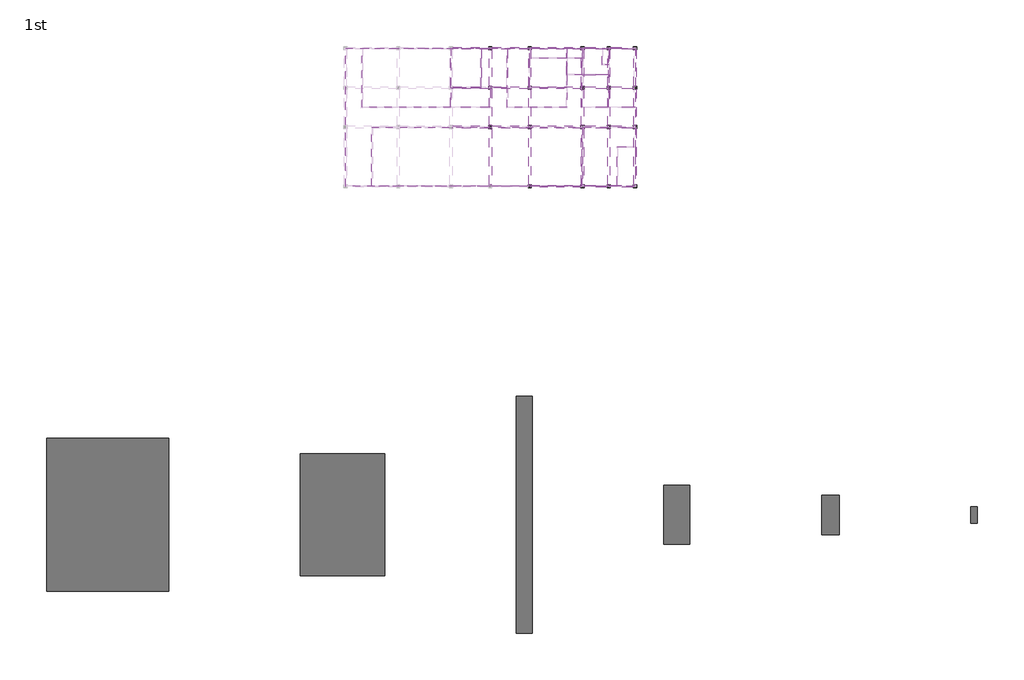
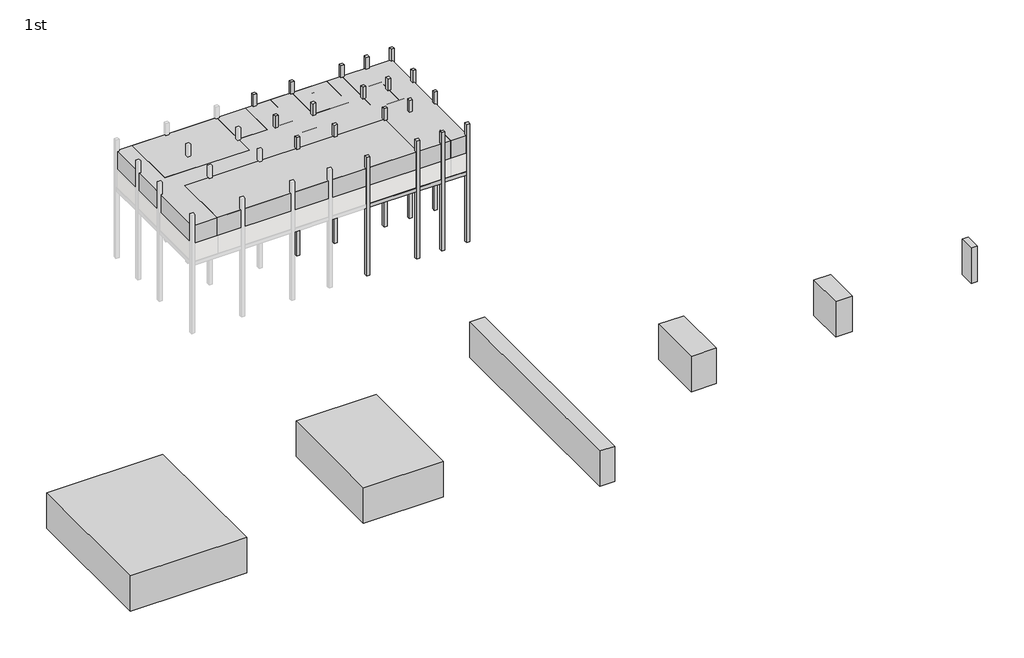
# One storey, part 3 of 3: 33 beams, 23 proxies, 19 columns.
"""IFC4 building model written with IfcOpenShell, lengths in millimetres."""

import ifcopenshell
import ifcopenshell.guid

model = None  # the IFC model being written
_history = None  # IfcOwnerHistory: only IFC2X3 demands one
_inside = {}  # id of a spatial element -> (the spatial element, [elements in it])
_under = {}  # id of a project, library or spatial element -> (it, [spatial elements below it])
_declared = {}  # id of a project -> (the project, [libraries it declares])
_typed = {}  # id of a type object -> (the type object, [elements of that type])
_made_of = {}  # id of a material, layer set ... -> (it, [elements and type objects made of it])


def new_model(schema):
    """Start an empty IFC model of exactly this schema.

    Asked for "IFC4X3", IfcOpenShell would pick the latest addendum, in which some entities
    have other attributes; the version numbers below select the first issue.
    IFC2X3 requires an IfcOwnerHistory on every rooted entity: one is made here for all.
    """
    global model, _history
    if schema == "IFC4X3":
        model = ifcopenshell.file(schema_version=(4, 3, 0, 0))
    else:
        model = ifcopenshell.file(schema=schema)
    _inside.clear()
    _under.clear()
    _declared.clear()
    _typed.clear()
    _made_of.clear()
    _history = None
    if model.schema == "IFC2X3":
        org = make("IfcOrganization", Name="unknown")
        user = make(
            "IfcPersonAndOrganization",
            ThePerson=make("IfcPerson", FamilyName="unknown"),
            TheOrganization=org,
        )
        app = make(
            "IfcApplication",
            ApplicationDeveloper=org,
            Version="unknown",
            ApplicationFullName="unknown",
            ApplicationIdentifier="unknown",
        )
        _history = make(
            "IfcOwnerHistory",
            OwningUser=user,
            OwningApplication=app,
            ChangeAction="ADDED",
            CreationDate=0,
        )
    return model


def make(cls, **values):
    """One entity of the class cls with the attributes given. An attribute that is None is left unset."""
    return model.create_entity(
        cls, **{name: value for name, value in values.items() if value is not None}
    )


def rooted(cls, **values):
    """An entity with a GlobalId (a new one), such as an element, a storey or a relation."""
    return make(cls, GlobalId=ifcopenshell.guid.new(), OwnerHistory=_history, **values)


def si_unit(unit_type, name, prefix=None):
    """IfcSIUnit, for example si_unit("LENGTHUNIT", "METRE", prefix="MILLI")."""
    return make("IfcSIUnit", UnitType=unit_type, Prefix=prefix, Name=name)


def assignment(units):
    """IfcUnitAssignment: the units of a project."""
    return None if units is None else make("IfcUnitAssignment", Units=units)


def point(xyz):
    """IfcCartesianPoint."""
    return None if xyz is None else make("IfcCartesianPoint", Coordinates=xyz)


def direction(xyz):
    """IfcDirection."""
    return None if xyz is None else make("IfcDirection", DirectionRatios=xyz)


def frame(location, z_axis=None, x_axis=None):
    """IfcAxis2Placement3D, a coordinate frame: its origin and axes. An axis left out is left unset."""
    return make(
        "IfcAxis2Placement3D",
        Location=point(location),
        Axis=direction(z_axis),
        RefDirection=direction(x_axis),
    )


def origin():
    """The frame at (0, 0, 0) with its axes left unset."""
    return frame((0.0, 0.0, 0.0))


def origin_with_axes():
    """The frame at (0, 0, 0) with the z axis (0, 0, 1) and the x axis (1, 0, 0) written out."""
    return frame((0.0, 0.0, 0.0), z_axis=(0.0, 0.0, 1.0), x_axis=(1.0, 0.0, 0.0))


def place(relative_to, where):
    """IfcLocalPlacement: puts the frame where relative to a parent placement (None: the world)."""
    return make(
        "IfcLocalPlacement", PlacementRelTo=relative_to, RelativePlacement=where
    )


def context(
    kind, dimensions, precision=None, world=None, true_north=None, identifier=None
):
    """IfcGeometricRepresentationContext, for example the 3D "Model" context."""
    return make(
        "IfcGeometricRepresentationContext",
        ContextIdentifier=identifier,
        ContextType=kind,
        CoordinateSpaceDimension=dimensions,
        Precision=precision,
        WorldCoordinateSystem=world,
        TrueNorth=true_north,
    )


def project(units=None, contexts=None):
    """IfcProject with its units and contexts."""
    return rooted(
        "IfcProject",
        Name="project",
        RepresentationContexts=contexts,
        UnitsInContext=assignment(units),
    )


def spatial(cls, under=None, at=None, **own):
    """A site, building, storey or space (cls), placed at a placement, below another one or the project."""
    s = rooted(cls, ObjectPlacement=at, **own)
    if under is not None:
        _under.setdefault(under.id(), (under, []))[1].append(s)
    return s


def polyline(points):
    """IfcPolyline through the points."""
    return make("IfcPolyline", Points=[point(p) for p in points])


def outline(outer, holes=None, kind="AREA"):
    """IfcArbitraryClosedProfileDef: a profile drawn as a closed curve; with holes, ...WithVoids."""
    if holes is None:
        return make("IfcArbitraryClosedProfileDef", ProfileType=kind, OuterCurve=outer)
    return make(
        "IfcArbitraryProfileDefWithVoids",
        ProfileType=kind,
        OuterCurve=outer,
        InnerCurves=holes,
    )


def extrude(swept, where, along, depth):
    """IfcExtrudedAreaSolid: the profile swept, set in the frame where, extruded along a direction by depth."""
    return make(
        "IfcExtrudedAreaSolid",
        SweptArea=swept,
        Position=where,
        ExtrudedDirection=direction(along),
        Depth=depth,
    )


def shape(context_of_items, identifier, shape_type, items):
    """IfcShapeRepresentation: the items that make up one representation, for example the "Body"."""
    return make(
        "IfcShapeRepresentation",
        ContextOfItems=context_of_items,
        RepresentationIdentifier=identifier,
        RepresentationType=shape_type,
        Items=items,
    )


def source(mapping_origin, context_of_items, identifier, shape_type, items):
    """IfcRepresentationMap: a shape defined once, which mapped items show again and again."""
    return make(
        "IfcRepresentationMap",
        MappingOrigin=mapping_origin,
        MappedRepresentation=shape(context_of_items, identifier, shape_type, items),
    )


def transform(
    local_origin,
    x_axis=None,
    y_axis=None,
    z_axis=None,
    scale=None,
    scale2=None,
    scale3=None,
    uniform=True,
):
    """IfcCartesianTransformationOperator3D, or its non-uniform kind. x_axis, y_axis, z_axis: its Axis1, 2, 3."""
    if uniform:
        return make(
            "IfcCartesianTransformationOperator3D",
            Axis1=direction(x_axis),
            Axis2=direction(y_axis),
            LocalOrigin=point(local_origin),
            Scale=scale,
            Axis3=direction(z_axis),
        )
    return make(
        "IfcCartesianTransformationOperator3DnonUniform",
        Axis1=direction(x_axis),
        Axis2=direction(y_axis),
        LocalOrigin=point(local_origin),
        Scale=scale,
        Axis3=direction(z_axis),
        Scale2=scale2,
        Scale3=scale3,
    )


def mapped(mapping_source, mapping_target):
    """IfcMappedItem: shows the shape of a source again, moved by a transform."""
    return make(
        "IfcMappedItem", MappingSource=mapping_source, MappingTarget=mapping_target
    )


def made_of(thing, what):
    """Note that an element or type object is made of a material, layer set ...; save() writes the relation."""
    if what is not None:
        _made_of.setdefault(what.id(), (what, []))[1].append(thing)
    return thing


def element(
    cls,
    number,
    at=None,
    inside=None,
    cuts=None,
    type_object=None,
    material=None,
    context=None,
    identifier="Body",
    shape_type=None,
    held_by="IfcProductDefinitionShape",
    body=None,
    shapes=None,
    **own,
):
    """One element of the class cls, such as IfcWall. Its Tag is "e" and its number.

    at: its placement. inside: the storey or other place that contains it. cuts: it is an
    opening in that element (IfcRelVoidsElement). A single representation is given by context,
    identifier, shape_type and body (its items); several are given by shapes. held_by: the class
    of the entity that holds the representations. save() writes the other relations.
    """
    e = rooted(cls, Tag="e%d" % number, ObjectPlacement=at, **own)
    if body is not None:
        shapes = [shape(context, identifier, shape_type, body)]
    if shapes is not None:
        e.Representation = make(held_by, Representations=shapes)
    if inside is not None:
        _inside.setdefault(inside.id(), (inside, []))[1].append(e)
    if cuts is not None:
        rooted(
            "IfcRelVoidsElement", RelatingBuildingElement=cuts, RelatedOpeningElement=e
        )
    if type_object is not None:
        _typed.setdefault(type_object.id(), (type_object, []))[1].append(e)
    return made_of(e, material)


def aggregate(whole, parts):
    """IfcRelAggregates: a whole, such as a stair, and the parts it consists of."""
    return rooted("IfcRelAggregates", RelatingObject=whole, RelatedObjects=parts)


def save(model, path):
    """Write the relations noted so far, then the file.

    IfcRelAggregates (storeys below a building ...), IfcRelContainedInSpatialStructure (elements
    in a storey), IfcRelDefinesByType, IfcRelAssociatesMaterial and IfcRelDeclares: one each for
    every whole, place, type object, material and project.
    """
    for whole, parts in _under.values():
        aggregate(whole, parts)
    for where, things in _inside.values():
        rooted(
            "IfcRelContainedInSpatialStructure",
            RelatedElements=things,
            RelatingStructure=where,
        )
    for kind, things in _typed.values():
        rooted("IfcRelDefinesByType", RelatedObjects=things, RelatingType=kind)
    for what, things in _made_of.values():
        rooted("IfcRelAssociatesMaterial", RelatedObjects=things, RelatingMaterial=what)
    for by, libraries in _declared.values():
        rooted("IfcRelDeclares", RelatingContext=by, RelatedDefinitions=libraries)
    model.write(path)


def generic_models_29bcd6f9(model_context):
    return source(origin(), model_context, "Body", "SweptSolid", [
        extrude(outline(polyline([(2000.0, 4500.0), (2000.0, -4500.0), (-2000.0, -4500.0), (-2000.0, 4500.0), (2000.0, 4500.0)])), origin_with_axes(), (0.0, 0.0, 1.0), 6000.0),
    ])


def generic_models_d82b1902(model_context):
    return source(origin(), model_context, "Body", "SweptSolid", [
        extrude(outline(polyline([(9300.0, 11600.0), (9300.0, -11600.0), (-9300.0, -11600.0), (-9300.0, 11600.0), (9300.0, 11600.0)])), origin_with_axes(), (0.0, 0.0, 1.0), 6000.0),
    ])


def generic_models_21711933(model_context):
    return source(origin(), model_context, "Body", "SweptSolid", [
        extrude(outline(polyline([(6400.0, 9300.0), (6400.0, -9300.0), (-6400.0, -9300.0), (-6400.0, 9300.0), (6400.0, 9300.0)])), origin_with_axes(), (0.0, 0.0, 1.0), 6000.0),
    ])


def generic_models_03d31222(model_context):
    return source(origin(), model_context, "Body", "SweptSolid", [
        extrude(outline(polyline([(1200.0, 18000.0), (1200.0, -18000.0), (-1200.0, -18000.0), (-1200.0, 18000.0), (1200.0, 18000.0)])), origin_with_axes(), (0.0, 0.0, 1.0), 6000.0),
    ])


def generic_models_5634f436(model_context):
    return source(origin(), model_context, "Body", "SweptSolid", [
        extrude(outline(polyline([(1350.0, 3000.0), (1350.0, -3000.0), (-1350.0, -3000.0), (-1350.0, 3000.0), (1350.0, 3000.0)])), origin_with_axes(), (0.0, 0.0, 1.0), 6000.0),
    ])


def generic_models_71e2440f(model_context):
    return source(origin(), model_context, "Body", "SweptSolid", [
        extrude(outline(polyline([(500.0, 1250.0), (500.0, -1250.0), (-500.0, -1250.0), (-500.0, 1250.0), (500.0, 1250.0)])), origin_with_axes(), (0.0, 0.0, 1.0), 6000.0),
    ])


def generic_models_57c7875f(model_context):
    return source(origin(), model_context, "Body", "SweptSolid", [
        extrude(outline(polyline([(4500.0, 16000.0), (4500.0, -16000.0), (-4500.0, -16000.0), (-4500.0, 16000.0), (4500.0, 16000.0)])), origin_with_axes(), (0.0, 0.0, 1.0), 6000.0),
    ])


def generic_models_7bff30ad(model_context):
    return source(origin(), model_context, "Body", "SweptSolid", [
        extrude(outline(polyline([(2000.0, 2000.0), (2000.0, -2000.0), (-2000.0, -2000.0), (-2000.0, 2000.0), (2000.0, 2000.0)])), origin_with_axes(), (0.0, 0.0, 1.0), 6000.0),
    ])


def generic_models_5b7b272c(model_context):
    return source(origin(), model_context, "Body", "SweptSolid", [
        extrude(outline(polyline([(2000.0, 2500.0), (2000.0, -2500.0), (-2000.0, -2500.0), (-2000.0, 2500.0), (2000.0, 2500.0)])), origin_with_axes(), (0.0, 0.0, 1.0), 6000.0),
    ])


def generic_models_47b98be1(model_context):
    return source(origin(), model_context, "Body", "SweptSolid", [
        extrude(outline(polyline([(1200.0, 2000.0), (1200.0, -2000.0), (-1200.0, -2000.0), (-1200.0, 2000.0), (1200.0, 2000.0)])), origin_with_axes(), (0.0, 0.0, 1.0), 6000.0),
    ])


def generic_models_7a053eeb(model_context):
    return source(origin(), model_context, "Body", "SweptSolid", [
        extrude(outline(polyline([(1200.0, 750.0), (1200.0, -750.0), (-1200.0, -750.0), (-1200.0, 750.0), (1200.0, 750.0)])), origin_with_axes(), (0.0, 0.0, 1.0), 6000.0),
    ])


def generic_models_ec17d728(model_context):
    return source(origin(), model_context, "Body", "SweptSolid", [
        extrude(outline(polyline([(2800.0, 3000.0), (2800.0, -3000.0), (-2800.0, -3000.0), (-2800.0, 3000.0), (2800.0, 3000.0)])), origin_with_axes(), (0.0, 0.0, 1.0), 6000.0),
    ])


def generic_models_85897e09(model_context):
    return source(origin(), model_context, "Body", "SweptSolid", [
        extrude(outline(polyline([(2800.0, 750.0), (2800.0, -750.0), (-2800.0, -750.0), (-2800.0, 750.0), (2800.0, 750.0)])), origin_with_axes(), (0.0, 0.0, 1.0), 6000.0),
    ])


def generic_models_b79df083(model_context):
    return source(origin(), model_context, "Body", "SweptSolid", [
        extrude(outline(polyline([(4500.0, 4500.0), (4500.0, -4500.0), (-4500.0, -4500.0), (-4500.0, 4500.0), (4500.0, 4500.0)])), origin_with_axes(), (0.0, 0.0, 1.0), 6000.0),
    ])


def generic_models_98b71764(model_context):
    return source(origin(), model_context, "Body", "SweptSolid", [
        extrude(outline(polyline([(2000.0, 3000.0), (2000.0, -3000.0), (-2000.0, -3000.0), (-2000.0, 3000.0), (2000.0, 3000.0)])), origin_with_axes(), (0.0, 0.0, 1.0), 6000.0),
    ])


def generic_models_1a87c0f4(model_context):
    return source(origin(), model_context, "Body", "SweptSolid", [
        extrude(outline(polyline([(2300.0, 3000.0), (2300.0, -3000.0), (-2300.0, -3000.0), (-2300.0, 3000.0), (2300.0, 3000.0)])), origin_with_axes(), (0.0, 0.0, 1.0), 6000.0),
    ])


def generic_models_df3bc381(model_context):
    return source(origin(), model_context, "Body", "SweptSolid", [
        extrude(outline(polyline([(4500.0, 6750.0), (4500.0, -6750.0), (-4500.0, -6750.0), (-4500.0, 6750.0), (4500.0, 6750.0)])), origin_with_axes(), (0.0, 0.0, 1.0), 6000.0),
    ])


def generic_models_542cc789(model_context):
    return source(origin(), model_context, "Body", "SweptSolid", [
        extrude(outline(polyline([(1500.0, 3000.0), (1500.0, -3000.0), (-1500.0, -3000.0), (-1500.0, 3000.0), (1500.0, 3000.0)])), origin_with_axes(), (0.0, 0.0, 1.0), 6000.0),
    ])


def generic_models_4d084078(model_context):
    return source(origin(), model_context, "Body", "SweptSolid", [
        extrude(outline(polyline([(4000.0, 4500.0), (4000.0, -4500.0), (-4000.0, -4500.0), (-4000.0, 4500.0), (4000.0, 4500.0)])), origin_with_axes(), (0.0, 0.0, 1.0), 6000.0),
    ])


def generic_models_7e8091d6(model_context):
    return source(origin(), model_context, "Body", "SweptSolid", [
        extrude(outline(polyline([(22000.0, 10500.0), (22000.0, -10500.0), (-22000.0, -10500.0), (-22000.0, 10500.0), (22000.0, 10500.0)])), origin_with_axes(), (0.0, 0.0, 1.0), 6000.0),
    ])


model = new_model("IFC4")

# Units and contexts
model_context = context("Model", 3, world=origin())
ifc_project = project(units=[si_unit("LENGTHUNIT", "METRE", prefix="MILLI")], contexts=[model_context])

# Site, building, storey
site = spatial("IfcSite", under=ifc_project)
building = spatial("IfcBuilding", under=site)
storey = spatial("IfcBuildingStorey", under=building, Name="1st", Elevation=6000.0)

# Beams
placement = place(None, origin())
element("IfcBeam", 1, ObjectType="Concrete-Rectangular-Beam : BM111_400x500_RG1", at=placement, inside=storey, context=model_context, shape_type="SweptSolid", body=[
    extrude(outline(polyline([(67284.6521483, 184673.8614395), (67634.6521483, 184673.8614395), (67634.6521483, 179173.8614395), (67284.6521483, 179173.8614395), (67284.6521483, 184673.8614395)])), frame((0.0, 0.0, 11400.0), z_axis=(0.0, 0.0, 1.0), x_axis=(1.0, 0.0, 0.0)), (0.0, 0.0, 1.0), 600.0),
])
element("IfcBeam", 2, ObjectType="Concrete-Rectangular-Beam : BM111_400x500_RG1", at=placement, inside=storey, context=model_context, shape_type="SweptSolid", body=[
    extrude(outline(polyline([(67284.6521483, 178673.8614395), (67634.6521483, 178673.8614395), (67634.6521483, 173173.8614395), (67284.6521483, 173173.8614395), (67284.6521483, 178673.8614395)])), frame((0.0, 0.0, 11400.0), z_axis=(0.0, 0.0, 1.0), x_axis=(1.0, 0.0, 0.0)), (0.0, 0.0, 1.0), 600.0),
])
element("IfcBeam", 3, ObjectType="Concrete-Rectangular-Beam : BM111_400x500_RG1", at=placement, inside=storey, context=model_context, shape_type="SweptSolid", body=[
    extrude(outline(polyline([(67284.6521483, 172673.8614395), (67634.6521483, 172673.8614395), (67634.6521483, 164173.8614395), (67284.6521483, 164173.8614395), (67284.6521483, 172673.8614395)])), frame((0.0, 0.0, 11400.0), z_axis=(0.0, 0.0, 1.0), x_axis=(1.0, 0.0, 0.0)), (0.0, 0.0, 1.0), 600.0),
])
element("IfcBeam", 4, ObjectType="Concrete-Rectangular-Beam : BM111_400x500_RG1", at=placement, inside=storey, context=model_context, shape_type="SweptSolid", body=[
    extrude(outline(polyline([(73284.6521483, 184673.8614395), (73634.6521483, 184673.8614395), (73634.6521483, 179173.8614395), (73284.6521483, 179173.8614395), (73284.6521483, 184673.8614395)])), frame((0.0, 0.0, 11400.0), z_axis=(0.0, 0.0, 1.0), x_axis=(1.0, 0.0, 0.0)), (0.0, 0.0, 1.0), 600.0),
])
element("IfcBeam", 5, ObjectType="Concrete-Rectangular-Beam : BM111_400x500_RG1", at=placement, inside=storey, context=model_context, shape_type="SweptSolid", body=[
    extrude(outline(polyline([(73284.6521483, 178673.8614395), (73634.6521483, 178673.8614395), (73634.6521483, 173173.8614395), (73284.6521483, 173173.8614395), (73284.6521483, 178673.8614395)])), frame((0.0, 0.0, 11400.0), z_axis=(0.0, 0.0, 1.0), x_axis=(1.0, 0.0, 0.0)), (0.0, 0.0, 1.0), 600.0),
])
element("IfcBeam", 6, ObjectType="Concrete-Rectangular-Beam : BM111_400x500_RG1", at=placement, inside=storey, context=model_context, shape_type="SweptSolid", body=[
    extrude(outline(polyline([(73284.6521483, 172673.8614395), (73634.6521483, 172673.8614395), (73634.6521483, 164173.8614395), (73284.6521483, 164173.8614395), (73284.6521483, 172673.8614395)])), frame((0.0, 0.0, 11400.0), z_axis=(0.0, 0.0, 1.0), x_axis=(1.0, 0.0, 0.0)), (0.0, 0.0, 1.0), 600.0),
])
element("IfcBeam", 7, ObjectType="Concrete-Rectangular-Beam : BM111_400x500_RG1", at=placement, inside=storey, context=model_context, shape_type="SweptSolid", body=[
    extrude(outline(polyline([(81284.6521483, 184673.8614395), (81634.6521483, 184673.8614395), (81634.6521483, 179173.8614395), (81284.6521483, 179173.8614395), (81284.6521483, 184673.8614395)])), frame((0.0, 0.0, 11400.0), z_axis=(0.0, 0.0, 1.0), x_axis=(1.0, 0.0, 0.0)), (0.0, 0.0, 1.0), 600.0),
])
element("IfcBeam", 8, ObjectType="Concrete-Rectangular-Beam : BM111_400x500_RG1", at=placement, inside=storey, context=model_context, shape_type="SweptSolid", body=[
    extrude(outline(polyline([(81284.6521483, 178673.8614395), (81634.6521483, 178673.8614395), (81634.6521483, 173173.8614395), (81284.6521483, 173173.8614395), (81284.6521483, 178673.8614395)])), frame((0.0, 0.0, 11400.0), z_axis=(0.0, 0.0, 1.0), x_axis=(1.0, 0.0, 0.0)), (0.0, 0.0, 1.0), 600.0),
])
element("IfcBeam", 9, ObjectType="Concrete-Rectangular-Beam : BM111_400x500_RG1", at=placement, inside=storey, context=model_context, shape_type="SweptSolid", body=[
    extrude(outline(polyline([(81284.6521483, 172673.8614395), (81634.6521483, 172673.8614395), (81634.6521483, 164173.8614395), (81284.6521483, 164173.8614395), (81284.6521483, 172673.8614395)])), frame((0.0, 0.0, 11400.0), z_axis=(0.0, 0.0, 1.0), x_axis=(1.0, 0.0, 0.0)), (0.0, 0.0, 1.0), 600.0),
])
element("IfcBeam", 10, ObjectType="Concrete-Rectangular-Beam : BM111_400x500_RG1", at=placement, inside=storey, context=model_context, shape_type="SweptSolid", body=[
    extrude(outline(polyline([(85284.6521483, 184673.8614395), (85634.6521483, 184673.8614395), (85634.6521483, 179173.8614395), (85284.6521483, 179173.8614395), (85284.6521483, 184673.8614395)])), frame((0.0, 0.0, 11400.0), z_axis=(0.0, 0.0, 1.0), x_axis=(1.0, 0.0, 0.0)), (0.0, 0.0, 1.0), 600.0),
])
element("IfcBeam", 11, ObjectType="Concrete-Rectangular-Beam : BM111_400x500_RG1", at=placement, inside=storey, context=model_context, shape_type="SweptSolid", body=[
    extrude(outline(polyline([(85284.6521483, 178673.8614395), (85634.6521483, 178673.8614395), (85634.6521483, 173173.8614395), (85284.6521483, 173173.8614395), (85284.6521483, 178673.8614395)])), frame((0.0, 0.0, 11400.0), z_axis=(0.0, 0.0, 1.0), x_axis=(1.0, 0.0, 0.0)), (0.0, 0.0, 1.0), 600.0),
])
element("IfcBeam", 12, ObjectType="Concrete-Rectangular-Beam : BM111_400x500_RG1", at=placement, inside=storey, context=model_context, shape_type="SweptSolid", body=[
    extrude(outline(polyline([(85284.6521483, 172673.8614395), (85634.6521483, 172673.8614395), (85634.6521483, 164173.8614395), (85284.6521483, 164173.8614395), (85284.6521483, 172673.8614395)])), frame((0.0, 0.0, 11400.0), z_axis=(0.0, 0.0, 1.0), x_axis=(1.0, 0.0, 0.0)), (0.0, 0.0, 1.0), 600.0),
])
element("IfcBeam", 13, ObjectType="Concrete-Rectangular-Beam : BM111_400x500_RG1", at=placement, inside=storey, context=model_context, shape_type="SweptSolid", body=[
    extrude(outline(polyline([(89284.6521483, 184673.8614395), (89634.6521483, 184673.8614395), (89634.6521483, 179173.8614395), (89284.6521483, 179173.8614395), (89284.6521483, 184673.8614395)])), frame((0.0, 0.0, 11400.0), z_axis=(0.0, 0.0, 1.0), x_axis=(1.0, 0.0, 0.0)), (0.0, 0.0, 1.0), 600.0),
])
element("IfcBeam", 14, ObjectType="Concrete-Rectangular-Beam : BM111_400x500_RG1", at=placement, inside=storey, context=model_context, shape_type="SweptSolid", body=[
    extrude(outline(polyline([(89284.6521483, 178673.8614395), (89634.6521483, 178673.8614395), (89634.6521483, 173173.8614395), (89284.6521483, 173173.8614395), (89284.6521483, 178673.8614395)])), frame((0.0, 0.0, 11400.0), z_axis=(0.0, 0.0, 1.0), x_axis=(1.0, 0.0, 0.0)), (0.0, 0.0, 1.0), 600.0),
])
element("IfcBeam", 15, ObjectType="Concrete-Rectangular-Beam : BM111_400x500_RG1", at=placement, inside=storey, context=model_context, shape_type="SweptSolid", body=[
    extrude(outline(polyline([(89284.6521483, 172673.8614395), (89634.6521483, 172673.8614395), (89634.6521483, 164173.8614395), (89284.6521483, 164173.8614395), (89284.6521483, 172673.8614395)])), frame((0.0, 0.0, 11400.0), z_axis=(0.0, 0.0, 1.0), x_axis=(1.0, 0.0, 0.0)), (0.0, 0.0, 1.0), 600.0),
])
element("IfcBeam", 16, ObjectType="Concrete-Rectangular-Beam : BM111_400x500_RG1", at=placement, inside=storey, context=model_context, shape_type="SweptSolid", body=[
    extrude(outline(polyline([(61709.6521483, 184748.8614395), (61709.6521483, 185098.8614395), (67209.6521483, 185098.8614395), (67209.6521483, 184748.8614395), (61709.6521483, 184748.8614395)])), frame((0.0, 0.0, 11400.0), z_axis=(0.0, 0.0, 1.0), x_axis=(1.0, 0.0, 0.0)), (0.0, 0.0, 1.0), 600.0),
])
element("IfcBeam", 17, ObjectType="Concrete-Rectangular-Beam : BM111_400x500_RG1", at=placement, inside=storey, context=model_context, shape_type="SweptSolid", body=[
    extrude(outline(polyline([(67709.6521483, 184748.8614395), (67709.6521483, 185098.8614395), (73209.6521483, 185098.8614395), (73209.6521483, 184748.8614395), (67709.6521483, 184748.8614395)])), frame((0.0, 0.0, 11400.0), z_axis=(0.0, 0.0, 1.0), x_axis=(1.0, 0.0, 0.0)), (0.0, 0.0, 1.0), 600.0),
])
element("IfcBeam", 18, ObjectType="Concrete-Rectangular-Beam : BM111_400x500_RG1", at=placement, inside=storey, context=model_context, shape_type="SweptSolid", body=[
    extrude(outline(polyline([(73709.6521483, 184748.8614395), (73709.6521483, 185098.8614395), (81209.6521483, 185098.8614395), (81209.6521483, 184748.8614395), (73709.6521483, 184748.8614395)])), frame((0.0, 0.0, 11400.0), z_axis=(0.0, 0.0, 1.0), x_axis=(1.0, 0.0, 0.0)), (0.0, 0.0, 1.0), 600.0),
])
element("IfcBeam", 19, ObjectType="Concrete-Rectangular-Beam : BM111_400x500_RG1", at=placement, inside=storey, context=model_context, shape_type="SweptSolid", body=[
    extrude(outline(polyline([(81709.6521483, 184748.8614395), (81709.6521483, 185098.8614395), (85209.6521483, 185098.8614395), (85209.6521483, 184748.8614395), (81709.6521483, 184748.8614395)])), frame((0.0, 0.0, 11400.0), z_axis=(0.0, 0.0, 1.0), x_axis=(1.0, 0.0, 0.0)), (0.0, 0.0, 1.0), 600.0),
])
element("IfcBeam", 20, ObjectType="Concrete-Rectangular-Beam : BM111_400x500_RG1", at=placement, inside=storey, context=model_context, shape_type="SweptSolid", body=[
    extrude(outline(polyline([(85709.6521483, 184748.8614395), (85709.6521483, 185098.8614395), (89209.6521483, 185098.8614395), (89209.6521483, 184748.8614395), (85709.6521483, 184748.8614395)])), frame((0.0, 0.0, 11400.0), z_axis=(0.0, 0.0, 1.0), x_axis=(1.0, 0.0, 0.0)), (0.0, 0.0, 1.0), 600.0),
])
element("IfcBeam", 21, ObjectType="Concrete-Rectangular-Beam : BM111_400x500_RG1", at=placement, inside=storey, context=model_context, shape_type="SweptSolid", body=[
    extrude(outline(polyline([(61709.6521483, 178748.8614395), (61709.6521483, 179098.8614395), (67209.6521483, 179098.8614395), (67209.6521483, 178748.8614395), (61709.6521483, 178748.8614395)])), frame((0.0, 0.0, 11400.0), z_axis=(0.0, 0.0, 1.0), x_axis=(1.0, 0.0, 0.0)), (0.0, 0.0, 1.0), 600.0),
])
element("IfcBeam", 22, ObjectType="Concrete-Rectangular-Beam : BM111_400x500_RG1", at=placement, inside=storey, context=model_context, shape_type="SweptSolid", body=[
    extrude(outline(polyline([(67709.6521483, 178748.8614395), (67709.6521483, 179098.8614395), (73209.6521483, 179098.8614395), (73209.6521483, 178748.8614395), (67709.6521483, 178748.8614395)])), frame((0.0, 0.0, 11400.0), z_axis=(0.0, 0.0, 1.0), x_axis=(1.0, 0.0, 0.0)), (0.0, 0.0, 1.0), 600.0),
])
element("IfcBeam", 23, ObjectType="Concrete-Rectangular-Beam : BM111_400x500_RG1", at=placement, inside=storey, context=model_context, shape_type="SweptSolid", body=[
    extrude(outline(polyline([(73709.6521483, 178748.8614395), (73709.6521483, 179098.8614395), (81209.6521483, 179098.8614395), (81209.6521483, 178748.8614395), (73709.6521483, 178748.8614395)])), frame((0.0, 0.0, 11400.0), z_axis=(0.0, 0.0, 1.0), x_axis=(1.0, 0.0, 0.0)), (0.0, 0.0, 1.0), 600.0),
])
element("IfcBeam", 24, ObjectType="Concrete-Rectangular-Beam : BM111_400x500_RG1", at=placement, inside=storey, context=model_context, shape_type="SweptSolid", body=[
    extrude(outline(polyline([(81709.6521483, 178748.8614395), (81709.6521483, 179098.8614395), (85209.6521483, 179098.8614395), (85209.6521483, 178748.8614395), (81709.6521483, 178748.8614395)])), frame((0.0, 0.0, 11400.0), z_axis=(0.0, 0.0, 1.0), x_axis=(1.0, 0.0, 0.0)), (0.0, 0.0, 1.0), 600.0),
])
element("IfcBeam", 25, ObjectType="Concrete-Rectangular-Beam : BM111_400x500_RG1", at=placement, inside=storey, context=model_context, shape_type="SweptSolid", body=[
    extrude(outline(polyline([(85709.6521483, 178748.8614395), (85709.6521483, 179098.8614395), (89209.6521483, 179098.8614395), (89209.6521483, 178748.8614395), (85709.6521483, 178748.8614395)])), frame((0.0, 0.0, 11400.0), z_axis=(0.0, 0.0, 1.0), x_axis=(1.0, 0.0, 0.0)), (0.0, 0.0, 1.0), 600.0),
])
element("IfcBeam", 26, ObjectType="Concrete-Rectangular-Beam : BM111_400x500_RG1", at=placement, inside=storey, context=model_context, shape_type="SweptSolid", body=[
    extrude(outline(polyline([(61709.6521483, 172748.8614395), (61709.6521483, 173098.8614395), (67209.6521483, 173098.8614395), (67209.6521483, 172748.8614395), (61709.6521483, 172748.8614395)])), frame((0.0, 0.0, 11400.0), z_axis=(0.0, 0.0, 1.0), x_axis=(1.0, 0.0, 0.0)), (0.0, 0.0, 1.0), 600.0),
])
element("IfcBeam", 27, ObjectType="Concrete-Rectangular-Beam : BM111_400x500_RG1", at=placement, inside=storey, context=model_context, shape_type="SweptSolid", body=[
    extrude(outline(polyline([(67709.6521483, 172748.8614395), (67709.6521483, 173098.8614395), (73209.6521483, 173098.8614395), (73209.6521483, 172748.8614395), (67709.6521483, 172748.8614395)])), frame((0.0, 0.0, 11400.0), z_axis=(0.0, 0.0, 1.0), x_axis=(1.0, 0.0, 0.0)), (0.0, 0.0, 1.0), 600.0),
])
element("IfcBeam", 28, ObjectType="Concrete-Rectangular-Beam : BM111_400x500_RG1", at=placement, inside=storey, context=model_context, shape_type="SweptSolid", body=[
    extrude(outline(polyline([(73709.6521483, 172748.8614395), (73709.6521483, 173098.8614395), (81209.6521483, 173098.8614395), (81209.6521483, 172748.8614395), (73709.6521483, 172748.8614395)])), frame((0.0, 0.0, 11400.0), z_axis=(0.0, 0.0, 1.0), x_axis=(1.0, 0.0, 0.0)), (0.0, 0.0, 1.0), 600.0),
])
element("IfcBeam", 29, ObjectType="Concrete-Rectangular-Beam : BM111_400x500_RG1", at=placement, inside=storey, context=model_context, shape_type="SweptSolid", body=[
    extrude(outline(polyline([(81709.6521483, 172748.8614395), (81709.6521483, 173098.8614395), (85209.6521483, 173098.8614395), (85209.6521483, 172748.8614395), (81709.6521483, 172748.8614395)])), frame((0.0, 0.0, 11400.0), z_axis=(0.0, 0.0, 1.0), x_axis=(1.0, 0.0, 0.0)), (0.0, 0.0, 1.0), 600.0),
])
element("IfcBeam", 30, ObjectType="Concrete-Rectangular-Beam : BM111_400x500_RG1", at=placement, inside=storey, context=model_context, shape_type="SweptSolid", body=[
    extrude(outline(polyline([(85709.6521483, 172748.8614395), (85709.6521483, 173098.8614395), (89209.6521483, 173098.8614395), (89209.6521483, 172748.8614395), (85709.6521483, 172748.8614395)])), frame((0.0, 0.0, 11400.0), z_axis=(0.0, 0.0, 1.0), x_axis=(1.0, 0.0, 0.0)), (0.0, 0.0, 1.0), 600.0),
])
element("IfcBeam", 31, ObjectType="Concrete-Rectangular-Beam : BM111_400x500_RG1", at=placement, inside=storey, context=model_context, shape_type="SweptSolid", body=[
    extrude(outline(polyline([(73709.6521483, 163748.8614395), (73709.6521483, 164098.8614395), (81209.6521483, 164098.8614395), (81209.6521483, 163748.8614395), (73709.6521483, 163748.8614395)])), frame((0.0, 0.0, 11400.0), z_axis=(0.0, 0.0, 1.0), x_axis=(1.0, 0.0, 0.0)), (0.0, 0.0, 1.0), 600.0),
])
element("IfcBeam", 32, ObjectType="Concrete-Rectangular-Beam : BM111_400x500_RG1", at=placement, inside=storey, context=model_context, shape_type="SweptSolid", body=[
    extrude(outline(polyline([(81709.6521483, 163748.8614395), (81709.6521483, 164098.8614395), (85209.6521483, 164098.8614395), (85209.6521483, 163748.8614395), (81709.6521483, 163748.8614395)])), frame((0.0, 0.0, 11400.0), z_axis=(0.0, 0.0, 1.0), x_axis=(1.0, 0.0, 0.0)), (0.0, 0.0, 1.0), 600.0),
])
element("IfcBeam", 33, ObjectType="Concrete-Rectangular-Beam : BM111_400x500_RG1", at=placement, inside=storey, context=model_context, shape_type="SweptSolid", body=[
    extrude(outline(polyline([(85709.6521483, 163748.8614395), (85709.6521483, 164098.8614395), (89209.6521483, 164098.8614395), (89209.6521483, 163748.8614395), (85709.6521483, 163748.8614395)])), frame((0.0, 0.0, 11400.0), z_axis=(0.0, 0.0, 1.0), x_axis=(1.0, 0.0, 0.0)), (0.0, 0.0, 1.0), 600.0),
])

# Proxies
generic_models_shape = generic_models_29bcd6f9(model_context)
element("IfcBuildingElementProxy", 34, Name="Space Planning Box_hec : Space Planning Box_hec", ObjectType="Space Planning Box_hec : Space Planning Box_hec", at=placement, inside=storey, context=model_context, shape_type="MappedRepresentation", body=[
    mapped(generic_models_shape, transform((95800.0, 114000.0, 6000.0), x_axis=(1.0, 0.0, 0.0), y_axis=(0.0, 1.0, 0.0), z_axis=(0.0, 0.0, 1.0))),
])
element("IfcBuildingElementProxy", 35, Name="Space Planning Box_hec : Space Planning Box_hec", ObjectType="Space Planning Box_hec : Space Planning Box_hec", at=placement, inside=storey, context=model_context, shape_type="MappedRepresentation", body=[
    mapped(generic_models_shape, transform((87459.6521483, 180423.8614395, 12000.0), x_axis=(1.0, 0.0, 0.0), y_axis=(0.0, 1.0, 0.0), z_axis=(0.0, 0.0, 1.0))),
])
generic_models_2_shape = generic_models_d82b1902(model_context)
element("IfcBuildingElementProxy", 36, Name="Space Planning Box_hec : Space Planning Box_hec", ObjectType="Space Planning Box_hec : Space Planning Box_hec", at=placement, inside=storey, context=model_context, shape_type="MappedRepresentation", body=[
    mapped(generic_models_2_shape, transform((9300.0, 114000.0, 6000.0), x_axis=(1.0, 0.0, 0.0), y_axis=(0.0, 1.0, 0.0), z_axis=(0.0, 0.0, 1.0))),
])
generic_models_3_shape = generic_models_21711933(model_context)
element("IfcBuildingElementProxy", 37, Name="Space Planning Box_hec : Space Planning Box_hec", ObjectType="Space Planning Box_hec : Space Planning Box_hec", at=placement, inside=storey, context=model_context, shape_type="MappedRepresentation", body=[
    mapped(generic_models_3_shape, transform((45000.0, 114000.0, 6000.0), x_axis=(1.0, 0.0, 0.0), y_axis=(0.0, 1.0, 0.0), z_axis=(0.0, 0.0, 1.0))),
])
generic_models_4_shape = generic_models_03d31222(model_context)
element("IfcBuildingElementProxy", 38, Name="Space Planning Box_hec : Space Planning Box_hec", ObjectType="Space Planning Box_hec : Space Planning Box_hec", at=placement, inside=storey, context=model_context, shape_type="MappedRepresentation", body=[
    mapped(generic_models_4_shape, transform((72600.0, 114000.0, 6000.0), x_axis=(1.0, 0.0, 0.0), y_axis=(0.0, 1.0, 0.0), z_axis=(0.0, 0.0, 1.0))),
])
generic_models_5_shape = generic_models_5634f436(model_context)
element("IfcBuildingElementProxy", 39, Name="Space Planning Box_hec : Space Planning Box_hec", ObjectType="Space Planning Box_hec : Space Planning Box_hec", at=placement, inside=storey, context=model_context, shape_type="MappedRepresentation", body=[
    mapped(generic_models_5_shape, transform((119150.0, 114000.0, 6000.0), x_axis=(1.0, 0.0, 0.0), y_axis=(0.0, 1.0, 0.0), z_axis=(0.0, 0.0, 1.0))),
])
element("IfcBuildingElementProxy", 40, Name="Space Planning Box_hec : Space Planning Box_hec", ObjectType="Space Planning Box_hec : Space Planning Box_hec", at=placement, inside=storey, context=model_context, shape_type="MappedRepresentation", body=[
    mapped(generic_models_5_shape, transform((88109.6521483, 166923.8614395, 12000.0), x_axis=(1.0, 0.0, 0.0), y_axis=(0.0, 1.0, 0.0), z_axis=(0.0, 0.0, 1.0))),
])
generic_models_6_shape = generic_models_71e2440f(model_context)
element("IfcBuildingElementProxy", 41, Name="Space Planning Box_hec : Space Planning Box_hec", ObjectType="Space Planning Box_hec : Space Planning Box_hec", at=placement, inside=storey, context=model_context, shape_type="MappedRepresentation", body=[
    mapped(generic_models_6_shape, transform((141000.0, 114000.0, 6000.0), x_axis=(1.0, 0.0, 0.0), y_axis=(0.0, 1.0, 0.0), z_axis=(0.0, 0.0, 1.0))),
])
element("IfcBuildingElementProxy", 42, Name="Space Planning Box_hec : Space Planning Box_hec", ObjectType="Space Planning Box_hec : Space Planning Box_hec", at=placement, inside=storey, context=model_context, shape_type="MappedRepresentation", body=[
    mapped(generic_models_6_shape, transform((84959.6521483, 183673.8614395, 12000.0), x_axis=(1.0, 0.0, 0.0), y_axis=(0.0, 1.0, 0.0), z_axis=(0.0, 0.0, 1.0))),
])
generic_models_7_shape = generic_models_57c7875f(model_context)
element("IfcBuildingElementProxy", 43, Name="Space Planning Box_hec : Space Planning Box_hec", ObjectType="Space Planning Box_hec : Space Planning Box_hec", at=placement, inside=storey, context=model_context, shape_type="MappedRepresentation", body=[
    mapped(generic_models_7_shape, transform((65459.6521483, 168423.8614395, 12000.0), x_axis=(0.0, -1.0, 0.0), y_axis=(1.0, 0.0, 0.0), z_axis=(0.0, 0.0, 1.0))),
])
generic_models_8_shape = generic_models_7bff30ad(model_context)
element("IfcBuildingElementProxy", 44, Name="Space Planning Box_hec : Space Planning Box_hec", ObjectType="Space Planning Box_hec : Space Planning Box_hec", at=placement, inside=storey, context=model_context, shape_type="MappedRepresentation", body=[
    mapped(generic_models_8_shape, transform((83459.6521483, 182923.8614395, 12000.0), x_axis=(1.0, 0.0, 0.0), y_axis=(0.0, 1.0, 0.0), z_axis=(0.0, 0.0, 1.0))),
])
generic_models_9_shape = generic_models_5b7b272c(model_context)
element("IfcBuildingElementProxy", 45, Name="Space Planning Box_hec : Space Planning Box_hec", ObjectType="Space Planning Box_hec : Space Planning Box_hec", at=placement, inside=storey, context=model_context, shape_type="MappedRepresentation", body=[
    mapped(generic_models_9_shape, transform((83459.6521483, 178423.8614395, 12000.0), x_axis=(1.0, 0.0, 0.0), y_axis=(0.0, 1.0, 0.0), z_axis=(0.0, 0.0, 1.0))),
])
generic_models_10_shape = generic_models_47b98be1(model_context)
element("IfcBuildingElementProxy", 46, Name="Space Planning Box_hec : Space Planning Box_hec", ObjectType="Space Planning Box_hec : Space Planning Box_hec", at=placement, inside=storey, context=model_context, shape_type="MappedRepresentation", body=[
    mapped(generic_models_10_shape, transform((80259.6521483, 182923.8614395, 12000.0), x_axis=(1.0, 0.0, 0.0), y_axis=(0.0, 1.0, 0.0), z_axis=(0.0, 0.0, 1.0))),
])
generic_models_11_shape = generic_models_7a053eeb(model_context)
element("IfcBuildingElementProxy", 47, Name="Space Planning Box_hec : Space Planning Box_hec", ObjectType="Space Planning Box_hec : Space Planning Box_hec", at=placement, inside=storey, context=model_context, shape_type="MappedRepresentation", body=[
    mapped(generic_models_11_shape, transform((80259.6521483, 184173.8614395, 12000.0), x_axis=(1.0, 0.0, 0.0), y_axis=(0.0, 1.0, 0.0), z_axis=(0.0, 0.0, 1.0))),
])
generic_models_12_shape = generic_models_ec17d728(model_context)
element("IfcBuildingElementProxy", 48, Name="Space Planning Box_hec : Space Planning Box_hec", ObjectType="Space Planning Box_hec : Space Planning Box_hec", at=placement, inside=storey, context=model_context, shape_type="MappedRepresentation", body=[
    mapped(generic_models_12_shape, transform((76259.6521483, 181923.8614395, 12000.0), x_axis=(1.0, 0.0, 0.0), y_axis=(0.0, 1.0, 0.0), z_axis=(0.0, 0.0, 1.0))),
])
generic_models_13_shape = generic_models_85897e09(model_context)
element("IfcBuildingElementProxy", 49, Name="Space Planning Box_hec : Space Planning Box_hec", ObjectType="Space Planning Box_hec : Space Planning Box_hec", at=placement, inside=storey, context=model_context, shape_type="MappedRepresentation", body=[
    mapped(generic_models_13_shape, transform((76259.6521483, 184173.8614395, 12000.0), x_axis=(1.0, 0.0, 0.0), y_axis=(0.0, 1.0, 0.0), z_axis=(0.0, 0.0, 1.0))),
])
generic_models_14_shape = generic_models_b79df083(model_context)
element("IfcBuildingElementProxy", 50, Name="Space Planning Box_hec : Space Planning Box_hec", ObjectType="Space Planning Box_hec : Space Planning Box_hec", at=placement, inside=storey, context=model_context, shape_type="MappedRepresentation", body=[
    mapped(generic_models_14_shape, transform((74559.6521483, 180423.8614395, 12000.0), x_axis=(1.0, 0.0, 0.0), y_axis=(0.0, 1.0, 0.0), z_axis=(0.0, 0.0, 1.0))),
])
generic_models_15_shape = generic_models_98b71764(model_context)
element("IfcBuildingElementProxy", 51, Name="Space Planning Box_hec : Space Planning Box_hec", ObjectType="Space Planning Box_hec : Space Planning Box_hec", at=placement, inside=storey, context=model_context, shape_type="MappedRepresentation", body=[
    mapped(generic_models_15_shape, transform((68059.6521483, 181923.8614395, 12000.0), x_axis=(1.0, 0.0, 0.0), y_axis=(0.0, 1.0, 0.0), z_axis=(0.0, 0.0, 1.0))),
])
generic_models_16_shape = generic_models_1a87c0f4(model_context)
element("IfcBuildingElementProxy", 52, Name="Space Planning Box_hec : Space Planning Box_hec", ObjectType="Space Planning Box_hec : Space Planning Box_hec", at=placement, inside=storey, context=model_context, shape_type="MappedRepresentation", body=[
    mapped(generic_models_16_shape, transform((63759.6521483, 181923.8614395, 12000.0), x_axis=(1.0, 0.0, 0.0), y_axis=(0.0, 1.0, 0.0), z_axis=(0.0, 0.0, 1.0))),
])
generic_models_17_shape = generic_models_df3bc381(model_context)
element("IfcBuildingElementProxy", 53, Name="Space Planning Box_hec : Space Planning Box_hec", ObjectType="Space Planning Box_hec : Space Planning Box_hec", at=placement, inside=storey, context=model_context, shape_type="MappedRepresentation", body=[
    mapped(generic_models_17_shape, transform((54709.6521483, 180423.8614395, 12000.0), x_axis=(0.0, -1.0, 0.0), y_axis=(1.0, 0.0, 0.0), z_axis=(0.0, 0.0, 1.0))),
])
generic_models_18_shape = generic_models_542cc789(model_context)
element("IfcBuildingElementProxy", 54, Name="Space Planning Box_hec : Space Planning Box_hec", ObjectType="Space Planning Box_hec : Space Planning Box_hec", at=placement, inside=storey, context=model_context, shape_type="MappedRepresentation", body=[
    mapped(generic_models_18_shape, transform((64459.6521483, 177423.8614395, 12000.0), x_axis=(0.0, -1.0, 0.0), y_axis=(1.0, 0.0, 0.0), z_axis=(0.0, 0.0, 1.0))),
])
generic_models_19_shape = generic_models_4d084078(model_context)
element("IfcBuildingElementProxy", 55, Name="Space Planning Box_hec : Space Planning Box_hec", ObjectType="Space Planning Box_hec : Space Planning Box_hec", at=placement, inside=storey, context=model_context, shape_type="MappedRepresentation", body=[
    mapped(generic_models_19_shape, transform((85459.6521483, 168423.8614395, 12000.0), x_axis=(1.0, 0.0, 0.0), y_axis=(0.0, 1.0, 0.0), z_axis=(0.0, 0.0, 1.0))),
])
generic_models_20_shape = generic_models_7e8091d6(model_context)
element("IfcBuildingElementProxy", 56, Name="Space Planning Box_hec : Space Planning Box_hec", ObjectType="Space Planning Box_hec : Space Planning Box_hec", at=placement, inside=storey, context=model_context, shape_type="MappedRepresentation", body=[
    mapped(generic_models_20_shape, transform((67459.6521483, 174423.8614395, 12000.0), x_axis=(1.0, 0.0, 0.0), y_axis=(0.0, 1.0, 0.0), z_axis=(0.0, 0.0, 1.0))),
])

# Columns
element("IfcColumn", 57, ObjectType="Concrete-Rectangular-Column : CL111_500x500", at=placement, inside=storey, context=model_context, shape_type="SweptSolid", body=[
    extrude(outline(polyline([(67709.6521483, 185173.8614395), (67709.6521483, 184673.8614395), (67209.6521483, 184673.8614395), (67209.6521483, 185173.8614395), (67709.6521483, 185173.8614395)])), origin_with_axes(), (0.0, 0.0, 1.0), 20000.0),
])
element("IfcColumn", 58, ObjectType="Concrete-Rectangular-Column : CL111_500x500", at=placement, inside=storey, context=model_context, shape_type="SweptSolid", body=[
    extrude(outline(polyline([(67709.6521483, 179173.8614395), (67709.6521483, 178673.8614395), (67209.6521483, 178673.8614395), (67209.6521483, 179173.8614395), (67709.6521483, 179173.8614395)])), origin_with_axes(), (0.0, 0.0, 1.0), 20000.0),
])
element("IfcColumn", 59, ObjectType="Concrete-Rectangular-Column : CL111_500x500", at=placement, inside=storey, context=model_context, shape_type="SweptSolid", body=[
    extrude(outline(polyline([(67709.6521483, 173173.8614395), (67709.6521483, 172673.8614395), (67209.6521483, 172673.8614395), (67209.6521483, 173173.8614395), (67709.6521483, 173173.8614395)])), origin_with_axes(), (0.0, 0.0, 1.0), 20000.0),
])
element("IfcColumn", 60, ObjectType="Concrete-Rectangular-Column : CL111_500x500", at=placement, inside=storey, context=model_context, shape_type="SweptSolid", body=[
    extrude(outline(polyline([(73709.6521483, 185173.8614395), (73709.6521483, 184673.8614395), (73209.6521483, 184673.8614395), (73209.6521483, 185173.8614395), (73709.6521483, 185173.8614395)])), origin_with_axes(), (0.0, 0.0, 1.0), 20000.0),
])
element("IfcColumn", 61, ObjectType="Concrete-Rectangular-Column : CL111_500x500", at=placement, inside=storey, context=model_context, shape_type="SweptSolid", body=[
    extrude(outline(polyline([(73709.6521483, 179173.8614395), (73709.6521483, 178673.8614395), (73209.6521483, 178673.8614395), (73209.6521483, 179173.8614395), (73709.6521483, 179173.8614395)])), origin_with_axes(), (0.0, 0.0, 1.0), 20000.0),
])
element("IfcColumn", 62, ObjectType="Concrete-Rectangular-Column : CL111_500x500", at=placement, inside=storey, context=model_context, shape_type="SweptSolid", body=[
    extrude(outline(polyline([(73709.6521483, 173173.8614395), (73709.6521483, 172673.8614395), (73209.6521483, 172673.8614395), (73209.6521483, 173173.8614395), (73709.6521483, 173173.8614395)])), origin_with_axes(), (0.0, 0.0, 1.0), 20000.0),
])
element("IfcColumn", 63, ObjectType="Concrete-Rectangular-Column : CL111_500x500", at=placement, inside=storey, context=model_context, shape_type="SweptSolid", body=[
    extrude(outline(polyline([(73709.6521483, 164173.8614395), (73709.6521483, 163673.8614395), (73209.6521483, 163673.8614395), (73209.6521483, 164173.8614395), (73709.6521483, 164173.8614395)])), origin_with_axes(), (0.0, 0.0, 1.0), 20000.0),
])
element("IfcColumn", 64, ObjectType="Concrete-Rectangular-Column : CL111_500x500", at=placement, inside=storey, context=model_context, shape_type="SweptSolid", body=[
    extrude(outline(polyline([(81709.6521483, 185173.8614395), (81709.6521483, 184673.8614395), (81209.6521483, 184673.8614395), (81209.6521483, 185173.8614395), (81709.6521483, 185173.8614395)])), origin_with_axes(), (0.0, 0.0, 1.0), 20000.0),
])
element("IfcColumn", 65, ObjectType="Concrete-Rectangular-Column : CL111_500x500", at=placement, inside=storey, context=model_context, shape_type="SweptSolid", body=[
    extrude(outline(polyline([(81709.6521483, 179173.8614395), (81709.6521483, 178673.8614395), (81209.6521483, 178673.8614395), (81209.6521483, 179173.8614395), (81709.6521483, 179173.8614395)])), origin_with_axes(), (0.0, 0.0, 1.0), 20000.0),
])
element("IfcColumn", 66, ObjectType="Concrete-Rectangular-Column : CL111_500x500", at=placement, inside=storey, context=model_context, shape_type="SweptSolid", body=[
    extrude(outline(polyline([(81709.6521483, 173173.8614395), (81709.6521483, 172673.8614395), (81209.6521483, 172673.8614395), (81209.6521483, 173173.8614395), (81709.6521483, 173173.8614395)])), origin_with_axes(), (0.0, 0.0, 1.0), 20000.0),
])
element("IfcColumn", 67, ObjectType="Concrete-Rectangular-Column : CL111_500x500", at=placement, inside=storey, context=model_context, shape_type="SweptSolid", body=[
    extrude(outline(polyline([(81709.6521483, 164173.8614395), (81709.6521483, 163673.8614395), (81209.6521483, 163673.8614395), (81209.6521483, 164173.8614395), (81709.6521483, 164173.8614395)])), origin_with_axes(), (0.0, 0.0, 1.0), 20000.0),
])
element("IfcColumn", 68, ObjectType="Concrete-Rectangular-Column : CL111_500x500", at=placement, inside=storey, context=model_context, shape_type="SweptSolid", body=[
    extrude(outline(polyline([(85709.6521483, 185173.8614395), (85709.6521483, 184673.8614395), (85209.6521483, 184673.8614395), (85209.6521483, 185173.8614395), (85709.6521483, 185173.8614395)])), origin_with_axes(), (0.0, 0.0, 1.0), 20000.0),
])
element("IfcColumn", 69, ObjectType="Concrete-Rectangular-Column : CL111_500x500", at=placement, inside=storey, context=model_context, shape_type="SweptSolid", body=[
    extrude(outline(polyline([(85709.6521483, 179173.8614395), (85709.6521483, 178673.8614395), (85209.6521483, 178673.8614395), (85209.6521483, 179173.8614395), (85709.6521483, 179173.8614395)])), origin_with_axes(), (0.0, 0.0, 1.0), 20000.0),
])
element("IfcColumn", 70, ObjectType="Concrete-Rectangular-Column : CL111_500x500", at=placement, inside=storey, context=model_context, shape_type="SweptSolid", body=[
    extrude(outline(polyline([(85709.6521483, 173173.8614395), (85709.6521483, 172673.8614395), (85209.6521483, 172673.8614395), (85209.6521483, 173173.8614395), (85709.6521483, 173173.8614395)])), origin_with_axes(), (0.0, 0.0, 1.0), 20000.0),
])
element("IfcColumn", 71, ObjectType="Concrete-Rectangular-Column : CL111_500x500", at=placement, inside=storey, context=model_context, shape_type="SweptSolid", body=[
    extrude(outline(polyline([(85709.6521483, 164173.8614395), (85709.6521483, 163673.8614395), (85209.6521483, 163673.8614395), (85209.6521483, 164173.8614395), (85709.6521483, 164173.8614395)])), origin_with_axes(), (0.0, 0.0, 1.0), 20000.0),
])
element("IfcColumn", 72, ObjectType="Concrete-Rectangular-Column : CL111_500x500", at=placement, inside=storey, context=model_context, shape_type="SweptSolid", body=[
    extrude(outline(polyline([(89709.6521483, 185173.8614395), (89709.6521483, 184673.8614395), (89209.6521483, 184673.8614395), (89209.6521483, 185173.8614395), (89709.6521483, 185173.8614395)])), origin_with_axes(), (0.0, 0.0, 1.0), 20000.0),
])
element("IfcColumn", 73, ObjectType="Concrete-Rectangular-Column : CL111_500x500", at=placement, inside=storey, context=model_context, shape_type="SweptSolid", body=[
    extrude(outline(polyline([(89709.6521483, 179173.8614395), (89709.6521483, 178673.8614395), (89209.6521483, 178673.8614395), (89209.6521483, 179173.8614395), (89709.6521483, 179173.8614395)])), origin_with_axes(), (0.0, 0.0, 1.0), 20000.0),
])
element("IfcColumn", 74, ObjectType="Concrete-Rectangular-Column : CL111_500x500", at=placement, inside=storey, context=model_context, shape_type="SweptSolid", body=[
    extrude(outline(polyline([(89709.6521483, 173173.8614395), (89709.6521483, 172673.8614395), (89209.6521483, 172673.8614395), (89209.6521483, 173173.8614395), (89709.6521483, 173173.8614395)])), origin_with_axes(), (0.0, 0.0, 1.0), 20000.0),
])
element("IfcColumn", 75, ObjectType="Concrete-Rectangular-Column : CL111_500x500", at=placement, inside=storey, context=model_context, shape_type="SweptSolid", body=[
    extrude(outline(polyline([(89709.6521483, 164173.8614395), (89709.6521483, 163673.8614395), (89209.6521483, 163673.8614395), (89209.6521483, 164173.8614395), (89709.6521483, 164173.8614395)])), origin_with_axes(), (0.0, 0.0, 1.0), 20000.0),
])

save(model, "model.ifc")

# Revit data of these elements
# Type "Concrete-Rectangular-Beam : BM111_400x500_RG1"
#   중앙부 하부근 = "3-D20"
#   중앙부 상부근 = "3-D20"
#   중앙부 보조근 = ""
#   중앙부 늑근 = "2-D10 @200"
#   외단부 하부근 = "3-D20"
#   외단부 상부근 = "3-D20"
#   외단부 보조근 = ""
#   외단부 늑근 = "2-D10 @100"
#   부호 = "RG1"
#   내단부 하부근 = "3-D20"
#   내단부 상부근 = "3-D20"
#   내단부 보조근 = ""
#   내단부 늑근 = "2-D10 @100"
#   ALL 하부근 = ""
#   ALL 상부근 = ""
#   ALL 보조근 = ""
#   ALL 늑근 = ""
#   Width = 400 mm
#   Height = 500 mm
#   Length [instance default] = 1524 mm
#   Structural Material [instance default] = 콘크리트 - 현장타설 콘크리트
#   hec_material3 [instance default] = none
#   hec_material2 [instance default] = none
#   hec_material1 [instance default] = none
#   Assembly Code = ""
# Type "Space Planning Box_hec : Space Planning Box_hec"
#   Type Comments = "..."
#   Room Name [instance default] = "?"
#   Interior Finish [instance default] = ""
#   Exterior Finish [instance default] = ""
#   Department [instance default] = ""
#   Assembly Code = "..."
#   Width [instance default] = 1524 mm
#   Program Area [instance default] = 0.00 m²
#   Length [instance default] = 1524 mm
#   Height [instance default] = 1524 mm
#   Area [instance default] = 2.32258 m²
#   Fill Color [instance default] = Cyan
#   Default Elevation = 0
# Type "Concrete-Rectangular-Column : CL111_500x500"
#   Description = "UG 철골 기둥용 Pedestal"
#   b = 500 mm
#   h = 500 mm
#   hec_material3 [instance default] = none
#   hec_material2 [instance default] = A03AE056-00001_Bitumen/Bituminous/Asphalt Coating
#   hec_material1 [instance default] = A03AC035-00001_Form Work (3 times in use)_Flat
#   Structural Material [instance default] = A03AC032-00007_Structural Concrete_Type1_25MPa-30Mpa
# Elements 1, 2, 3, 4, 5, 6, 7, 8, 9, 10, 11, 12, 13, 14, 15, 16, 17, 18, 19, 20, 21, 22, 23, 24, 25, 26, 27, 28, 29, 30, 31, 32, 33 (IfcBeam, "Concrete-Rectangular-Beam : BM111_400x500_RG1")
#   Comments = ""
#   hec_material3 = none
#   hec_material2 = none
#   hec_material1 = none
#   Structural Material = 콘크리트 - 현장타설 콘크리트
#   Phase Created = New Construction
#   Materials on its faces: "콘크리트 - 현장타설 콘크리트"
# Element 34 (IfcBuildingElementProxy, "Space Planning Box_hec : Space Planning Box_hec")
#   Room Name = "Stairway"
#   Interior Finish = "IF2"
#   Exterior Finish = "EF1"
#   Department = "AR"
#   Width = 4000 mm
#   Program Area = 36.00 m²
#   Length = 9000 mm
#   Height = 6000 mm
#   Area = 36.00 m²
#   Fill Color = Lavender
#   Phase Created = New Construction
#   Materials on its faces: "Lavender"
# Element 35 (IfcBuildingElementProxy, "Space Planning Box_hec : Space Planning Box_hec")
#   Room Name = "Stairway"
#   Interior Finish = "IF2"
#   Exterior Finish = "EF1"
#   Department = "AR"
#   Width = 4000 mm
#   Program Area = 38.00 m²
#   Length = 9000 mm
#   Height = 6000 mm
#   Area = 36.00 m²
#   Fill Color = Lavender
#   Phase Created = New Construction
#   Materials on its faces: "Lavender"
# Element 36 (IfcBuildingElementProxy, "Space Planning Box_hec : Space Planning Box_hec")
#   Room Name = "Electronic Room"
#   Interior Finish = "IF1"
#   Exterior Finish = "EF1"
#   Department = "CI"
#   Width = 18600 mm
#   Program Area = 431.52 m²
#   Length = 23200 mm
#   Height = 6000 mm
#   Area = 431.52 m²
#   Fill Color = Lime
#   Phase Created = New Construction
#   Materials on its faces: "Lime"
# Element 37 (IfcBuildingElementProxy, "Space Planning Box_hec : Space Planning Box_hec")
#   Room Name = "Electrical Room"
#   Interior Finish = "IF1"
#   Exterior Finish = "EF1"
#   Department = "EL"
#   Width = 12800 mm
#   Program Area = 238.08 m²
#   Length = 18600 mm
#   Height = 6000 mm
#   Area = 238.08 m²
#   Fill Color = Blue
#   Phase Created = New Construction
#   Materials on its faces: "Blue"
# Element 38 (IfcBuildingElementProxy, "Space Planning Box_hec : Space Planning Box_hec")
#   Room Name = "Corridor"
#   Interior Finish = "IF2-1"
#   Exterior Finish = "EF1"
#   Department = "AR"
#   Width = 2400 mm
#   Program Area = 86.40 m²
#   Length = 36000 mm
#   Height = 6000 mm
#   Area = 86.40 m²
#   Fill Color = Lavender
#   Phase Created = New Construction
#   Materials on its faces: "Lavender"
# Elements 39, 40 (IfcBuildingElementProxy, "Space Planning Box_hec : Space Planning Box_hec")
#   Room Name = "Duct Shaft"
#   Interior Finish = "NA"
#   Exterior Finish = "EF1"
#   Department = "HV"
#   Width = 2700 mm
#   Program Area = 16.20 m²
#   Length = 6000 mm
#   Height = 6000 mm
#   Area = 16.20 m²
#   Fill Color = Pink
#   Phase Created = New Construction
#   Materials on its faces: "Pink"
# Elements 41, 42 (IfcBuildingElementProxy, "Space Planning Box_hec : Space Planning Box_hec")
#   Room Name = "Pipe Shaft"
#   Interior Finish = "NA"
#   Exterior Finish = "EF1"
#   Department = "HV"
#   Width = 1000 mm
#   Program Area = 2.50 m²
#   Length = 2500 mm
#   Height = 6000 mm
#   Area = 2.50 m²
#   Fill Color = Pink
#   Phase Created = New Construction
#   Materials on its faces: "Pink"
# Element 43 (IfcBuildingElementProxy, "Space Planning Box_hec : Space Planning Box_hec")
#   Room Name = "Central Control Room"
#   Interior Finish = "IF3"
#   Exterior Finish = "EF1"
#   Department = "CI"
#   Width = 9000 mm
#   Program Area = 288.00 m²
#   Length = 32000 mm
#   Height = 6000 mm
#   Area = 288.00 m²
#   Fill Color = Lime
#   Phase Created = New Construction
#   Materials on its faces: "Lime"
# Element 44 (IfcBuildingElementProxy, "Space Planning Box_hec : Space Planning Box_hec")
#   Room Name = "Toilet (F)"
#   Interior Finish = "IF5"
#   Exterior Finish = "EF1"
#   Department = "AR"
#   Width = 4000 mm
#   Program Area = 72.00 m²
#   Length = 4000 mm
#   Height = 6000 mm
#   Area = 16.00 m²
#   Fill Color = Lavender
#   Phase Created = New Construction
#   Materials on its faces: "Lavender"
# Element 45 (IfcBuildingElementProxy, "Space Planning Box_hec : Space Planning Box_hec")
#   Room Name = "Toilet (M)"
#   Interior Finish = "IF5"
#   Exterior Finish = "EF1"
#   Department = "AR"
#   Width = 4000 mm
#   Program Area = 72.00 m²
#   Length = 5000 mm
#   Height = 6000 mm
#   Area = 20.00 m²
#   Fill Color = Lavender
#   Phase Created = New Construction
#   Materials on its faces: "Lavender"
# Element 46 (IfcBuildingElementProxy, "Space Planning Box_hec : Space Planning Box_hec")
#   Room Name = "Locker Room (F)"
#   Interior Finish = "IF2-1"
#   Exterior Finish = "EF1"
#   Department = "AR"
#   Width = 2400 mm
#   Program Area = 31.50 m²
#   Length = 4000 mm
#   Height = 6000 mm
#   Area = 9.60 m²
#   Fill Color = Lavender
#   Phase Created = New Construction
#   Materials on its faces: "Lavender"
# Element 47 (IfcBuildingElementProxy, "Space Planning Box_hec : Space Planning Box_hec")
#   Room Name = "Shower Room (F)"
#   Interior Finish = "IF5"
#   Exterior Finish = "EF1"
#   Department = "AR"
#   Width = 2400 mm
#   Program Area = 31.50 m²
#   Length = 1500 mm
#   Height = 6000 mm
#   Area = 3.60 m²
#   Fill Color = Lavender
#   Phase Created = New Construction
#   Materials on its faces: "Lavender"
# Element 48 (IfcBuildingElementProxy, "Space Planning Box_hec : Space Planning Box_hec")
#   Room Name = "Locker Room (M)"
#   Interior Finish = "IF2-1"
#   Exterior Finish = "EF1"
#   Department = "AR"
#   Width = 5600 mm
#   Program Area = 31.50 m²
#   Length = 6000 mm
#   Height = 6000 mm
#   Area = 33.60 m²
#   Fill Color = Lavender
#   Phase Created = New Construction
#   Materials on its faces: "Lavender"
# Element 49 (IfcBuildingElementProxy, "Space Planning Box_hec : Space Planning Box_hec")
#   Room Name = "Shower Room (M)"
#   Interior Finish = "IF5"
#   Exterior Finish = "EF1"
#   Department = "AR"
#   Width = 5600 mm
#   Program Area = 31.50 m²
#   Length = 1500 mm
#   Height = 6000 mm
#   Area = 8.40 m²
#   Fill Color = Lavender
#   Phase Created = New Construction
#   Materials on its faces: "Lavender"
# Element 50 (IfcBuildingElementProxy, "Space Planning Box_hec : Space Planning Box_hec")
#   Room Name = "Kitch & Lunch Room"
#   Interior Finish = "IF2-1"
#   Exterior Finish = "EF1"
#   Department = "AR"
#   Width = 9000 mm
#   Program Area = 31.50 m²
#   Length = 9000 mm
#   Height = 6000 mm
#   Area = 81.00 m²
#   Fill Color = Lavender
#   Phase Created = New Construction
#   Materials on its faces: "Lavender"
# Element 51 (IfcBuildingElementProxy, "Space Planning Box_hec : Space Planning Box_hec")
#   Room Name = "Shift Office Room"
#   Interior Finish = "IF2-1"
#   Exterior Finish = "EF1"
#   Department = "AR"
#   Width = 4000 mm
#   Program Area = 43.20 m²
#   Length = 6000 mm
#   Height = 6000 mm
#   Area = 24.00 m²
#   Fill Color = Lavender
#   Phase Created = New Construction
#   Materials on its faces: "Lavender"
# Element 52 (IfcBuildingElementProxy, "Space Planning Box_hec : Space Planning Box_hec")
#   Room Name = "Document Room"
#   Interior Finish = "IF2-1"
#   Exterior Finish = "EF1"
#   Department = "AR"
#   Width = 4600 mm
#   Program Area = 48.00 m²
#   Length = 6000 mm
#   Height = 6000 mm
#   Area = 27.60 m²
#   Fill Color = Lavender
#   Phase Created = New Construction
#   Materials on its faces: "Lavender"
# Element 53 (IfcBuildingElementProxy, "Space Planning Box_hec : Space Planning Box_hec")
#   Room Name = "Engineer Room"
#   Interior Finish = "IF3"
#   Exterior Finish = "EF1"
#   Department = "CI"
#   Width = 9000 mm
#   Program Area = 120.00 m²
#   Length = 13500 mm
#   Height = 6000 mm
#   Area = 121.50 m²
#   Fill Color = Lime
#   Phase Created = New Construction
#   Materials on its faces: "Lime"
# Element 54 (IfcBuildingElementProxy, "Space Planning Box_hec : Space Planning Box_hec")
#   Room Name = "LOTO Office Room"
